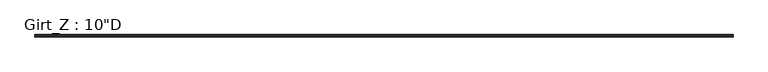
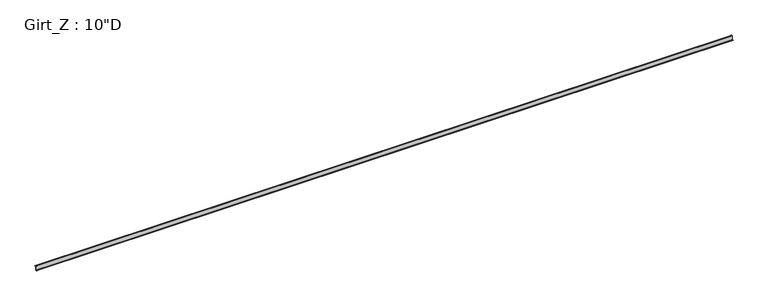
"""IFC4 building model written with IfcOpenShell, lengths in millimetres: beam geometry."""

from ifc_helpers import new_model, si_unit, point, frame, frame_2d, origin, place, context, project, spatial, polyline, circle_curve, trimmed, segment, composite_curve, outline, extrude, source, transform, mapped, element, save


def beam_95257211(model_context):
    return source(origin(), model_context, "Body", "SweptSolid", [
        extrude(outline(composite_curve([segment(polyline([(63.5, 127.0), (75.745104, 112.4068534), (73.6169367, 110.621109), (62.204539, 124.221875), (3.3005807, 124.221875)]), True, "CONTINUOUS"), segment(trimmed(circle_curve(frame_2d((3.3741066, 122.2381931)), 1.9850441), [point((3.3005807, 124.221875))], [point((1.3890625, 122.2381931))], True, "CARTESIAN"), True, "CONTINUOUS"), segment(polyline([(1.3890625, 122.2381931), (1.3890625, -122.2375)]), True, "CONTINUOUS"), segment(trimmed(circle_curve(frame_2d((-3.3734375, -122.2375)), 4.7625), [point((1.3890625, -122.2375))], [point((-3.3734375, -127.0))], False, "CARTESIAN"), True, "CONTINUOUS"), segment(polyline([(-3.3734375, -127.0), (-63.5, -127.0), (-75.745104, -112.4068534), (-73.6169367, -110.621109), (-62.204539, -124.221875), (-3.2694106, -124.221875)]), True, "CONTINUOUS"), segment(trimmed(circle_curve(frame_2d((-3.3748024, -122.2389339)), 1.9857399), [point((-3.2694106, -124.221875))], [point((-1.3890625, -122.2389339))], True, "CARTESIAN"), True, "CONTINUOUS"), segment(polyline([(-1.3890625, -122.2389339), (-1.3890625, 122.2375)]), True, "CONTINUOUS"), segment(trimmed(circle_curve(frame_2d((3.3734375, 122.2375)), 4.7625), [point((-1.3890625, 122.2375))], [point((3.3734375, 127.0))], False, "CARTESIAN"), True, "CONTINUOUS"), segment(polyline([(3.3734375, 127.0), (63.5, 127.0)]), True, "CONTINUOUS")], self_intersect=False)), frame((-21165.82, 0.0, 0.0), z_axis=(1.0, 0.0, 0.0), x_axis=(0.0, 1.0, 0.0)), (0.0, 0.0, 1.0), 42331.64),
    ])


if __name__ == "__main__":
    model = new_model("IFC4")
    model_context = context("Model", 3, world=origin())
    ifc_project = project(units=[si_unit("LENGTHUNIT", "METRE", prefix="MILLI")], contexts=[model_context])
    site = spatial("IfcSite", under=ifc_project)
    building = spatial("IfcBuilding", under=site)
    placement = place(None, origin())
    beam_shape = beam_95257211(model_context)
    element("IfcBeam", 1, ObjectType="Girt_Z : 10\"D", at=placement, inside=building, context=model_context, shape_type="MappedRepresentation", body=[
        mapped(beam_shape, transform((0.0, 0.0, 0.0), x_axis=(1.0, 0.0, 0.0), y_axis=(0.0, 1.0, 0.0), z_axis=(0.0, 0.0, 1.0))),
    ])
    save(model, "model.ifc")

# Revit data of these elements
# Type "Girt_Z : 10\"D"
#   Web_Thickness = 0' - 0 7/64"
#   Length [instance default] = 10' - 0"
#   Leg_1 = 0' - 2 1/2"
#   Height = 0' - 10"
#   Structural Material [instance default] = none
# Element 1 (IfcBeam, "Girt_Z : 10\"D")
#   Structural Material = Steel
#   Materials on its faces: "Steel"
# Materials
#   "Steel": class "Metal", colour RGB 118 118 114, transparency 0, Description = "Steel, mill finish", Cost = 0
